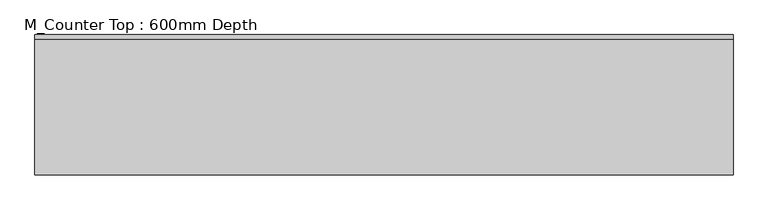
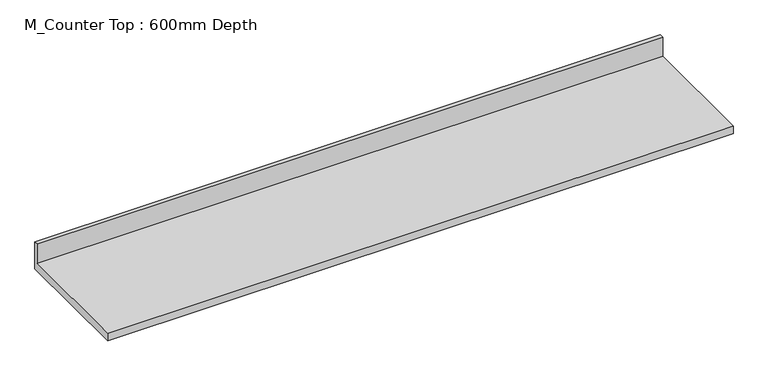
"""IFC4 building model written with IfcOpenShell, lengths in millimetres: furniture geometry, M_Counter Top : 600mm Depth."""

from ifc_helpers import new_model, si_unit, frame, origin, place, context, project, spatial, polyline, outline, extrude, source, transform, mapped, element, save


def m_counter_top_600mm_depth_2414b025(model_context):
    return source(origin(), model_context, "Body", "SweptSolid", [
        extrude(outline(polyline([(0.0, 1001.6), (0.0, 860.0), (-625.0, 860.0), (-625.0, 900.0), (-19.05, 900.0), (-19.05, 1001.6), (0.0, 1001.6)])), frame((-1200.4622951, 0.0, 0.0), z_axis=(1.0, 0.0, 0.0), x_axis=(0.0, 1.0, 0.0)), (0.0, 0.0, 1.0), 3109.1000242),
    ])


if __name__ == "__main__":
    model = new_model("IFC4")
    model_context = context("Model", 3, world=origin())
    ifc_project = project(units=[si_unit("LENGTHUNIT", "METRE", prefix="MILLI")], contexts=[model_context])
    site = spatial("IfcSite", under=ifc_project)
    building = spatial("IfcBuilding", under=site)
    placement = place(None, origin())
    m_counter_top_600mm_depth_shape = m_counter_top_600mm_depth_2414b025(model_context)
    element("IfcFurniture", 1, ObjectType="M_Counter Top : 600mm Depth", at=placement, inside=building, context=model_context, shape_type="MappedRepresentation", body=[
        mapped(m_counter_top_600mm_depth_shape, transform((0.0, 0.0, 0.0), x_axis=(1.0, 0.0, 0.0), y_axis=(0.0, 1.0, 0.0), z_axis=(0.0, 0.0, 1.0))),
    ])
    save(model, "model.ifc")

# Revit data of these elements
# Type "M_Counter Top : 600mm Depth"
#   COBie.Type.CreatedBy = "design@eagle.com"
#   COBie.Type.CreatedOn = "2016-09-01T06:50:21"
#   COBie.Type.Name = "Casework_M_Counter Top_600mm Depth"
#   COBie.Type.Category = "23-40 35 17 47 11 : Kitchen Casework"
#   COBie.Type.Description = ""
#   COBie.Type.Manufacturer = ""
#   COBie.Type.ModelNumber = ""
#   COBie.Type.ReplacementCost = 0
#   Counter Thickness = 40 mm
#   Depth = 625 mm
#   Height = 900 mm
#   Length [instance default] = 2500 mm
#   COBie.Type = no
#   Counter Top Material = none
# Element 1 (IfcFurniture, "M_Counter Top : 600mm Depth")
#   Length = 3109.1 mm
#   Materials on its faces: "Counter Top"
# Materials
#   "Counter Top": class "Wood", colour RGB 226 177 128, transparency 0
